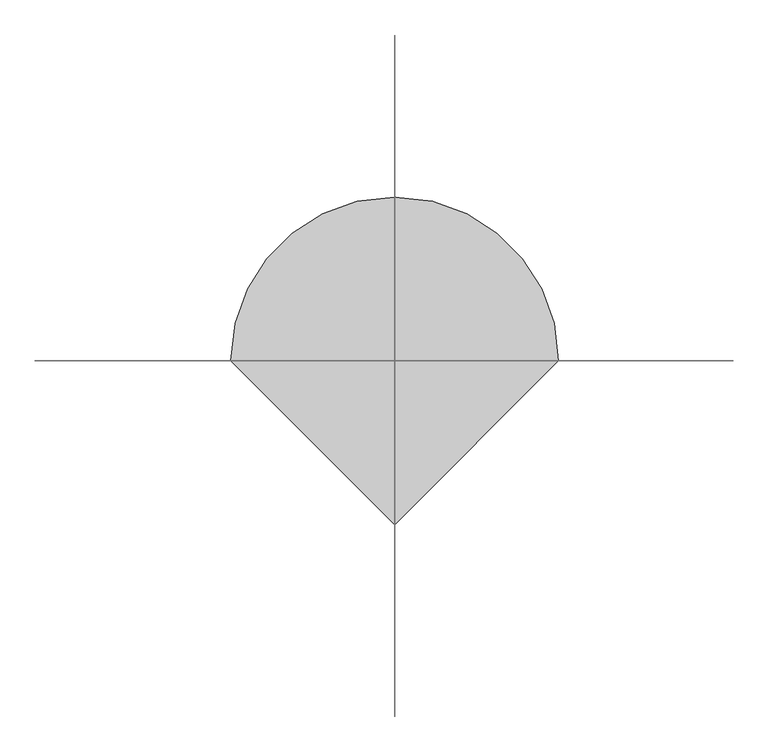
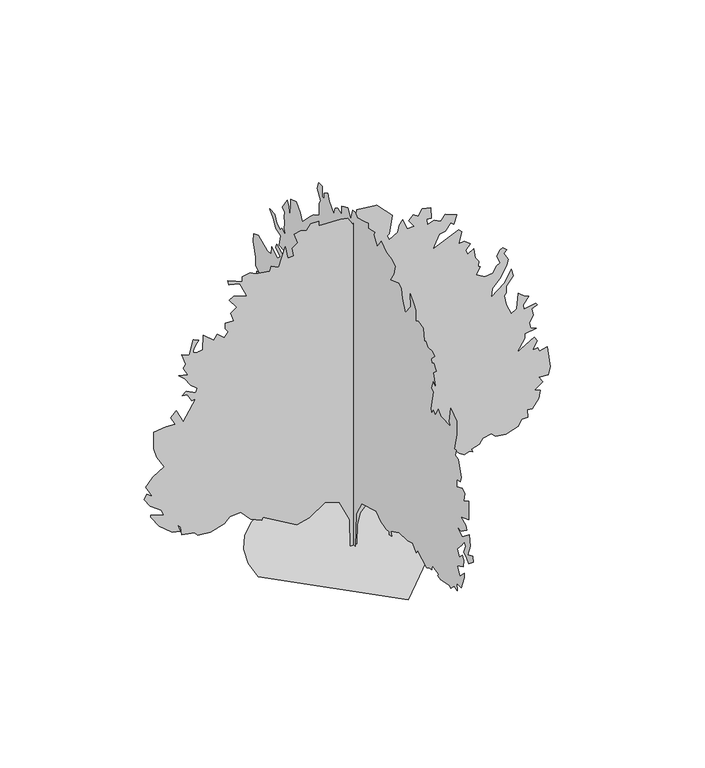
"""IFC4 building model written with IfcOpenShell, lengths in millimetres: proxy geometry, daphne 26070 : daphne 26070."""

import ifcopenshell
import ifcopenshell.guid

model = None  # the IFC model being written
_history = None  # IfcOwnerHistory: only IFC2X3 demands one
_inside = {}  # id of a spatial element -> (the spatial element, [elements in it])
_under = {}  # id of a project, library or spatial element -> (it, [spatial elements below it])
_declared = {}  # id of a project -> (the project, [libraries it declares])
_typed = {}  # id of a type object -> (the type object, [elements of that type])
_made_of = {}  # id of a material, layer set ... -> (it, [elements and type objects made of it])


def new_model(schema):
    """Start an empty IFC model of exactly this schema.

    Asked for "IFC4X3", IfcOpenShell would pick the latest addendum, in which some entities
    have other attributes; the version numbers below select the first issue.
    IFC2X3 requires an IfcOwnerHistory on every rooted entity: one is made here for all.
    """
    global model, _history
    if schema == "IFC4X3":
        model = ifcopenshell.file(schema_version=(4, 3, 0, 0))
    else:
        model = ifcopenshell.file(schema=schema)
    _inside.clear()
    _under.clear()
    _declared.clear()
    _typed.clear()
    _made_of.clear()
    _history = None
    if model.schema == "IFC2X3":
        org = make("IfcOrganization", Name="unknown")
        user = make(
            "IfcPersonAndOrganization",
            ThePerson=make("IfcPerson", FamilyName="unknown"),
            TheOrganization=org,
        )
        app = make(
            "IfcApplication",
            ApplicationDeveloper=org,
            Version="unknown",
            ApplicationFullName="unknown",
            ApplicationIdentifier="unknown",
        )
        _history = make(
            "IfcOwnerHistory",
            OwningUser=user,
            OwningApplication=app,
            ChangeAction="ADDED",
            CreationDate=0,
        )
    return model


def make(cls, **values):
    """One entity of the class cls with the attributes given. An attribute that is None is left unset."""
    return model.create_entity(
        cls, **{name: value for name, value in values.items() if value is not None}
    )


def rooted(cls, **values):
    """An entity with a GlobalId (a new one), such as an element, a storey or a relation."""
    return make(cls, GlobalId=ifcopenshell.guid.new(), OwnerHistory=_history, **values)


def si_unit(unit_type, name, prefix=None):
    """IfcSIUnit, for example si_unit("LENGTHUNIT", "METRE", prefix="MILLI")."""
    return make("IfcSIUnit", UnitType=unit_type, Prefix=prefix, Name=name)


def assignment(units):
    """IfcUnitAssignment: the units of a project."""
    return None if units is None else make("IfcUnitAssignment", Units=units)


def point(xyz):
    """IfcCartesianPoint."""
    return None if xyz is None else make("IfcCartesianPoint", Coordinates=xyz)


def direction(xyz):
    """IfcDirection."""
    return None if xyz is None else make("IfcDirection", DirectionRatios=xyz)


def frame(location, z_axis=None, x_axis=None):
    """IfcAxis2Placement3D, a coordinate frame: its origin and axes. An axis left out is left unset."""
    return make(
        "IfcAxis2Placement3D",
        Location=point(location),
        Axis=direction(z_axis),
        RefDirection=direction(x_axis),
    )


def origin():
    """The frame at (0, 0, 0) with its axes left unset."""
    return frame((0.0, 0.0, 0.0))


def place(relative_to, where):
    """IfcLocalPlacement: puts the frame where relative to a parent placement (None: the world)."""
    return make(
        "IfcLocalPlacement", PlacementRelTo=relative_to, RelativePlacement=where
    )


def context(
    kind, dimensions, precision=None, world=None, true_north=None, identifier=None
):
    """IfcGeometricRepresentationContext, for example the 3D "Model" context."""
    return make(
        "IfcGeometricRepresentationContext",
        ContextIdentifier=identifier,
        ContextType=kind,
        CoordinateSpaceDimension=dimensions,
        Precision=precision,
        WorldCoordinateSystem=world,
        TrueNorth=true_north,
    )


def project(units=None, contexts=None):
    """IfcProject with its units and contexts."""
    return rooted(
        "IfcProject",
        Name="project",
        RepresentationContexts=contexts,
        UnitsInContext=assignment(units),
    )


def spatial(cls, under=None, at=None, **own):
    """A site, building, storey or space (cls), placed at a placement, below another one or the project."""
    s = rooted(cls, ObjectPlacement=at, **own)
    if under is not None:
        _under.setdefault(under.id(), (under, []))[1].append(s)
    return s


def point_list(points):
    """IfcCartesianPointList2D or 3D."""
    cls = (
        "IfcCartesianPointList2D" if len(points[0]) == 2 else "IfcCartesianPointList3D"
    )
    return make(cls, CoordList=points)


def triangles(points, corners, closed=None, point_numbers=None):
    """IfcTriangulatedFaceSet: each triangle names its three corners, points numbered from 1."""
    return make(
        "IfcTriangulatedFaceSet",
        Coordinates=point_list(points),
        Closed=closed,
        CoordIndex=corners,
        PnIndex=point_numbers,
    )


def shape(context_of_items, identifier, shape_type, items):
    """IfcShapeRepresentation: the items that make up one representation, for example the "Body"."""
    return make(
        "IfcShapeRepresentation",
        ContextOfItems=context_of_items,
        RepresentationIdentifier=identifier,
        RepresentationType=shape_type,
        Items=items,
    )


def source(mapping_origin, context_of_items, identifier, shape_type, items):
    """IfcRepresentationMap: a shape defined once, which mapped items show again and again."""
    return make(
        "IfcRepresentationMap",
        MappingOrigin=mapping_origin,
        MappedRepresentation=shape(context_of_items, identifier, shape_type, items),
    )


def transform(
    local_origin,
    x_axis=None,
    y_axis=None,
    z_axis=None,
    scale=None,
    scale2=None,
    scale3=None,
    uniform=True,
):
    """IfcCartesianTransformationOperator3D, or its non-uniform kind. x_axis, y_axis, z_axis: its Axis1, 2, 3."""
    if uniform:
        return make(
            "IfcCartesianTransformationOperator3D",
            Axis1=direction(x_axis),
            Axis2=direction(y_axis),
            LocalOrigin=point(local_origin),
            Scale=scale,
            Axis3=direction(z_axis),
        )
    return make(
        "IfcCartesianTransformationOperator3DnonUniform",
        Axis1=direction(x_axis),
        Axis2=direction(y_axis),
        LocalOrigin=point(local_origin),
        Scale=scale,
        Axis3=direction(z_axis),
        Scale2=scale2,
        Scale3=scale3,
    )


def mapped(mapping_source, mapping_target):
    """IfcMappedItem: shows the shape of a source again, moved by a transform."""
    return make(
        "IfcMappedItem", MappingSource=mapping_source, MappingTarget=mapping_target
    )


def made_of(thing, what):
    """Note that an element or type object is made of a material, layer set ...; save() writes the relation."""
    if what is not None:
        _made_of.setdefault(what.id(), (what, []))[1].append(thing)
    return thing


def element(
    cls,
    number,
    at=None,
    inside=None,
    cuts=None,
    type_object=None,
    material=None,
    context=None,
    identifier="Body",
    shape_type=None,
    held_by="IfcProductDefinitionShape",
    body=None,
    shapes=None,
    **own,
):
    """One element of the class cls, such as IfcWall. Its Tag is "e" and its number.

    at: its placement. inside: the storey or other place that contains it. cuts: it is an
    opening in that element (IfcRelVoidsElement). A single representation is given by context,
    identifier, shape_type and body (its items); several are given by shapes. held_by: the class
    of the entity that holds the representations. save() writes the other relations.
    """
    e = rooted(cls, Tag="e%d" % number, ObjectPlacement=at, **own)
    if body is not None:
        shapes = [shape(context, identifier, shape_type, body)]
    if shapes is not None:
        e.Representation = make(held_by, Representations=shapes)
    if inside is not None:
        _inside.setdefault(inside.id(), (inside, []))[1].append(e)
    if cuts is not None:
        rooted(
            "IfcRelVoidsElement", RelatingBuildingElement=cuts, RelatedOpeningElement=e
        )
    if type_object is not None:
        _typed.setdefault(type_object.id(), (type_object, []))[1].append(e)
    return made_of(e, material)


def aggregate(whole, parts):
    """IfcRelAggregates: a whole, such as a stair, and the parts it consists of."""
    return rooted("IfcRelAggregates", RelatingObject=whole, RelatedObjects=parts)


def save(model, path):
    """Write the relations noted so far, then the file.

    IfcRelAggregates (storeys below a building ...), IfcRelContainedInSpatialStructure (elements
    in a storey), IfcRelDefinesByType, IfcRelAssociatesMaterial and IfcRelDeclares: one each for
    every whole, place, type object, material and project.
    """
    for whole, parts in _under.values():
        aggregate(whole, parts)
    for where, things in _inside.values():
        rooted(
            "IfcRelContainedInSpatialStructure",
            RelatedElements=things,
            RelatingStructure=where,
        )
    for kind, things in _typed.values():
        rooted("IfcRelDefinesByType", RelatedObjects=things, RelatingType=kind)
    for what, things in _made_of.values():
        rooted("IfcRelAssociatesMaterial", RelatedObjects=things, RelatingMaterial=what)
    for by, libraries in _declared.values():
        rooted("IfcRelDeclares", RelatingContext=by, RelatedDefinitions=libraries)
    model.write(path)


def entourage_98a115af(model_context):
    return source(origin(), model_context, "Body", "Tessellation", [
        triangles([(-9.4573925, 3.9e-06, 72.2348623), (-36.4693492, 6.1e-06, 128.8771626), (-74.629579, 5.2e-06, 141.2324949), (-113.9485589, 1.8e-06, 114.0498972), (-145.9624841, -1e-07, 106.0463523), (-234.001251, -8e-07, 158.0691489), (-236.002001, -1.4e-06, 150.0658583), (-264.0154255, -1.9e-06, 162.0709213), (-290.0250479, -1.3e-06, 190.0833467), (-318.0387268, -2.7e-06, 188.0823242), (-332.0443036, -4.1e-06, 174.0762387), (-368.4272936, -6.4e-06, 163.6409018), (-400.0731817, -7.6e-06, 166.0726938), (-408.0767266, -7.3e-06, 176.0772612), (-442.0924192, -8.5e-06, 182.0797836), (-444.0939686, -7.2e-06, 204.089414), (-452.0975135, -7.1e-06, 212.0929589), (-446.0929381, -7.9e-06, 194.0851191), (-466.1030903, -8.6e-06, 198.0868916), (-500.1187829, -8.4e-06, 226.0990444), (-522.1279046, -7.4e-06, 258.1124609), (-522.1279046, -7.1e-06, 264.1170363), (-488.1121757, -6.3e-06, 252.1104472), (-494.1142076, -5.6e-06, 268.117537), (-522.9229142, -5.6e-06, 288.9353979), (-538.1349944, -4.9e-06, 312.1357804), (-532.1304191, -3.9e-06, 324.1423513), (-518.1248423, -3.9e-06, 314.1372934), (-534.1319321, -2.8e-06, 344.14996), (-516.6084741, -8e-07, 365.2878413), (-486.7989927, 1.6e-06, 383.4742676), (-506.1208148, 2.7e-06, 416.1818642), (-514.1243597, 3.9e-06, 442.1940482), (-514.1243597, 6.5e-06, 486.2122553), (-482.1101801, 8.1e-06, 490.2153176), (-458.099509, 9.1e-06, 488.2138046), (-470.1035728, 9.9e-06, 510.2229263), (-456.097996, 1.13e-05, 524.2284668), (-438.0893932, 1e-05, 488.2138046), (-406.0752136, 1.45e-05, 540.2355566), (-416.0802715, 1.39e-05, 538.236587), (-428.0868788, 1.46e-05, 558.2441957), (-440.0909062, 1.42e-05, 560.2457088), (-430.0883918, 1.51e-05, 568.2492537), (-406.0752136, 1.54e-05, 556.2426827), (-401.4955876, 1.62e-05, 567.0275259), (-418.0817845, 1.63e-05, 580.2533175), (-434.0888743, 1.7e-05, 604.2639522), (-450.0959641, 1.72e-05, 618.2720724), (-426.0853294, 1.79e-05, 612.2674971), (-438.0893932, 1.87e-05, 634.2791622), (-432.0873613, 1.94e-05, 642.2826708), (-442.0924192, 2.07e-05, 672.2953737), (-422.0823034, 2.11e-05, 664.2917925), (-412.0797526, 2.38e-05, 702.308004), (-398.0716687, 2.41e-05, 696.3059721), (-400.6802304, 2.38e-05, 693.2783226), (-403.212634, 2.35e-05, 690.2023476), (-405.5926123, 2.32e-05, 687.0248526), (-407.7439708, 2.29e-05, 683.6948959), (-409.5930948, 2.26e-05, 680.1642975), (-411.0637536, 2.23e-05, 676.3821882), (-412.0797526, 2.21e-05, 672.2953737), (-411.9857903, 2.19e-05, 668.7317104), (-410.3525688, 2.18e-05, 666.420369), (-407.434106, 2.18e-05, 665.1452288), (-403.4920137, 2.2e-05, 664.7033226), (-398.7777666, 2.22e-05, 664.8861603), (-393.5530128, 2.25e-05, 665.485615), (-388.0691179, 2.28e-05, 666.2907984), (-386.0676049, 2.52e-05, 706.3085592), (-360.0554572, 2.49e-05, 682.2978882), (-350.0529064, 2.62e-05, 696.3059721), (-332.0443036, 2.6e-05, 680.2988823), (-322.0392457, 2.72e-05, 692.3029461), (-330.0427906, 2.76e-05, 704.3095533), (-330.0427906, 2.84e-05, 718.3150938), (-308.0336689, 2.94e-05, 718.3150938), (-316.0372138, 3.03e-05, 740.3242155), (-301.0029389, 3.16e-05, 751.5637184), (-320.0377327, 3.24e-05, 778.340427), (-308.0336689, 3.33e-05, 784.3424589), (-274.0179581, 3.42e-05, 774.3399445), (-292.0265791, 3.57e-05, 812.356156), (-320.9191106, 3.49e-05, 820.7254852), (-324.0407587, 3.54e-05, 832.3637283), (-304.0306247, 3.58e-05, 824.3602198), (-286.0245472, 3.62e-05, 816.3566385), (-286.0245472, 3.7e-05, 830.3647951), (-265.0619096, 3.8e-05, 832.6329706), (-252.0090908, 3.82e-05, 826.3616964), (-215.9931387, 3.95e-05, 820.3596645), (-211.9913662, 4.03e-05, 832.3637283), (-191.9827583, 4.06e-05, 822.3612139), (-175.9756504, 4.43e-05, 872.3814892), (-168.7203883, 4.27e-05, 839.3385933), (-153.9660381, 4.34e-05, 840.3673096), (-157.9678106, 4.45e-05, 862.3789747), (-143.9617251, 4.57e-05, 872.3814892), (-151.9650156, 4.69e-05, 898.3936369), (-135.9581802, 4.78e-05, 902.3941195), (-119.9513447, 4.83e-05, 898.3936369), (-109.9467864, 4.96e-05, 912.3991774), (-89.9381694, 5.05e-05, 912.3991774), (-89.9381694, 4.97e-05, 900.3951862), (-32.626833, 5.21e-05, 897.7739073), (-14.3439498, 5.26e-05, 893.5625364), (-1.8993678, 5.19e-05, 872.3814892), (6.1041838, 5.31e-05, 886.3895731), (8.105045, 5.45e-05, 908.3986948), (59.627565, 5.65e-05, 903.8140182), (99.4230465, 5.58e-05, 862.5999641), (92.1418776, 5.26e-05, 814.3577053), (86.1393461, 5.21e-05, 810.3546066), (92.1418776, 5.16e-05, 798.3505428), (114.1514989, 5.33e-05, 810.3546066), (118.1578496, 5.45e-05, 827.9416145), (126.1568253, 5.56e-05, 840.3673096), (138.1621427, 5.45e-05, 812.356156), (155.7905089, 5.52e-05, 811.8684677), (142.1639151, 5.58e-05, 832.3637283), (154.1689872, 5.71e-05, 844.3703356), (166.1743046, 5.71e-05, 836.3667543), (176.1785995, 5.85e-05, 852.3739168), (198.1884842, 5.92e-05, 848.3708181), (200.188998, 5.75e-05, 818.3581879), (188.1839168, 5.71e-05, 820.3596645), (190.1846849, 5.63e-05, 804.3525747), (208.1927972, 5.74e-05, 810.3546066), (224.199887, 5.76e-05, 802.3510981), (236.20495, 5.9e-05, 816.3566385), (265.7807247, 5.96e-05, 805.7293076), (258.2140718, 5.79e-05, 782.343453), (250.2110355, 5.79e-05, 788.3454849), (236.20495, 5.62e-05, 770.3369184), (220.1978602, 5.54e-05, 768.3379126), (204.1910248, 5.26e-05, 732.3207069), (270.2206608, 5.73e-05, 762.3333372), (278.2242057, 5.71e-05, 754.3298286), (270.2206608, 5.5e-05, 724.3171257), (284.2262195, 5.57e-05, 726.318675), (300.2333274, 5.57e-05, 714.3120678), (288.2267384, 5.43e-05, 700.3065273), (294.2312955, 5.39e-05, 688.3024635), (309.737998, 5.51e-05, 697.179756), (312.8444218, 5.37e-05, 671.3504459), (322.242431, 5.33e-05, 658.2872171), (320.240918, 5.25e-05, 646.283226), (326.2454933, 5.25e-05, 642.2801273), (316.2403991, 5.1e-05, 624.2741043), (337.7847236, 5.12e-05, 610.9797123), (358.2596729, 5.23e-05, 614.2690464), (368.2621874, 5.37e-05, 630.2761362), (378.0386619, 5.44e-05, 634.7135107), (368.2621874, 5.52e-05, 656.2882839), (376.2657323, 5.64e-05, 670.2938244), (384.2692772, 5.7e-05, 674.2943069), (394.2743714, 5.68e-05, 664.2917925), (386.2708265, 5.61e-05, 658.2872171), (398.1707179, 5.54e-05, 637.1290609), (394.2743714, 5.43e-05, 622.272555), (376.2657323, 5.17e-05, 592.2598884), (356.2581599, 4.97e-05, 572.2497725), (354.2566106, 4.83e-05, 550.2406508), (388.2723395, 5.13e-05, 576.2527986), (406.2783989, 5.4e-05, 608.2669782), (410.2814612, 5.3e-05, 588.2568624), (392.2728221, 5.09e-05, 566.2477407), (392.2728221, 4.98e-05, 548.2391015), (388.2723395, 4.93e-05, 542.2371059), (392.2728221, 4.79e-05, 516.2249219), (406.2783989, 4.67e-05, 486.2122553), (419.6692966, 4.79e-05, 495.1530613), (424.2870017, 5.05e-05, 536.235074), (440.2941278, 5.04e-05, 522.2294972), (450.2991858, 5.06e-05, 518.2264712), (437.047996, 4.89e-05, 500.1924339), (438.2925785, 4.83e-05, 488.2138046), (468.3077886, 4.99e-05, 494.2158002), (472.3083075, 4.97e-05, 488.2138046), (458.3027307, 4.88e-05, 482.2117727), (462.5902596, 4.78e-05, 462.3895815), (452.3006988, 4.64e-05, 446.1945308), (456.3012177, 4.56e-05, 430.187441), (470.3067581, 4.58e-05, 424.1854091), (440.2941278, 4.43e-05, 420.1849265), (440.2941278, 4.36e-05, 408.1783193), (420.2865191, 4.08e-05, 376.1641397), (464.3047626, 4.43e-05, 402.1762874), (472.3083075, 4.39e-05, 390.1697165), (460.3017002, 4.21e-05, 368.1605947), (474.3098205, 4.28e-05, 370.1621078), (478.3103394, 4.24e-05, 360.1570498), (498.3204552, 4.35e-05, 364.1600759), (506.3240001, 4.05e-05, 308.1352615), (500.3194247, 3.9e-05, 288.1251276), (476.3113335, 3.81e-05, 290.1266587), (486.3138843, 3.76e-05, 274.1195508), (464.3047626, 3.57e-05, 258.1124609), (480.3118524, 3.6e-05, 252.1104472), (476.3113335, 3.47e-05, 232.1015668), (460.3017002, 3.26e-05, 210.0919546), (446.2961234, 3.22e-05, 212.0929589), (448.2976727, 3.09e-05, 190.0833467), (432.2905829, 3.02e-05, 190.0833467), (424.2870017, 2.89e-05, 174.0762387), (391.7419679, 2.69e-05, 164.3614974), (366.2632178, 2.6e-05, 168.0737163), (354.2566106, 2.61e-05, 178.0780111), (332.2474889, 2.49e-05, 174.0762387), (323.8020015, 2.37e-05, 160.8723026), (302.2348404, 2.24e-05, 154.0673764), (306.2353412, 2.21e-05, 146.0640859), (298.2317963, 2.2e-05, 150.0658583), (284.2262195, 2.11e-05, 146.0640859), (272.2196304, 2.11e-05, 154.0673764), (260.2155848, 2.14e-05, 168.0737163), (240.2064682, 2.03e-05, 164.0719438), (236.8051496, 1.96e-05, 155.3752181), (196.1874799, 1.67e-05, 136.0595276), (196.1874799, 1.6e-05, 124.0544646), (162.1725321, 1.36e-05, 110.0481247), (162.1725321, 1.4e-05, 116.0509106), (138.1618883, 1.27e-05, 112.0491381), (106.7192036, 1.23e-05, 127.7984221), (83.214788, 1.13e-05, 128.4156446), (38.7434109, 8e-06, 104.983363), (17.3291135, 5.6e-06, 81.0641653), (9.1189377, 3.5e-06, 51.8726831), (8.1050195, 4e-07, 0.0), (-7.9020227, -3e-07, 7e-07), (-244.9072532, 0.0, 4.54e-05), (-238.4327937, 56.1165193, 4.18e-05), (-219.9933851, 107.6506239, 3.79e-05), (-191.0655541, 153.1257915, 3.39e-05), (-153.1257915, 191.0655541, 3e-05), (-107.6506239, 219.9933851, 2.63e-05), (-56.1165193, 238.4327937, 2.29e-05), (1.14e-05, 244.9072532, 2.01e-05), (56.1165193, 238.4327937, 1.8e-05), (107.6506239, 219.9933851, 5.12e-05), (153.1257915, 191.0655541, 5.1e-05), (191.0655541, 153.1257915, 5.16e-05), (219.9933851, 107.6506239, 1.87e-05), (238.4327937, 56.1165193, 2.09e-05), (244.9072532, -2.14e-05, 2.4e-05), (-3.16e-05, -244.9072532, 4.93e-05), (-1e-06, 8.7682648, 19.1210077), (-2.7e-06, 9.3654196, 78.8180451), (-6.1e-06, 33.2534526, 124.0544646), (-5.1e-06, 45.2590243, 110.0481247), (-5.2e-06, 55.2633328, 118.0516787), (-5.8e-06, 63.2666234, 112.0491381), (-6.9e-06, 91.2787853, 114.0498972), (-9e-06, 105.285116, 130.0569961), (-9.8e-06, 121.2919515, 126.0552236), (-9.6e-06, 133.2972779, 144.0630725), (-1.09e-05, 133.2972779, 162.0709213), (-1.16e-05, 181.318293, 146.0640859), (-1.37e-05, 187.3210879, 152.0666174), (-1.51e-05, 221.3357813, 154.0676308), (-1.31e-05, 215.3334951, 146.0640859), (-1.58e-05, 241.3446436, 158.0694032), (-1.53e-05, 243.3454117, 172.0754887), (-1.59e-05, 257.3504617, 172.0754887), (-1.75e-05, 259.3519928, 188.0825785), (-1.71e-05, 267.3555377, 204.089414), (-1.9e-05, 271.3585819, 214.0939814), (-1.92e-05, 297.3682044, 236.1036118), (-2.09e-05, 291.3661725, 240.1051299), (-2.09e-05, 315.3768253, 264.1170363), (-2.19e-05, 325.3818832, 250.1096791), (-2.19e-05, 331.3839151, 256.1134914), (-2.32e-05, 351.394031, 248.1086748), (-2.37e-05, 357.3960629, 242.1061342), (-2.46e-05, 381.4066976, 244.1069023), (-2.44e-05, 385.4072165, 254.1119602), (-2.53e-05, 409.4178512, 258.1124609), (-2.69e-05, 411.4193642, 272.1180377), (-2.71e-05, 423.423428, 278.1225949), (-2.96e-05, 455.4376076, 302.1332478), (-2.88e-05, 443.4335438, 310.1367745), (-3.05e-05, 469.4457278, 346.151473), (-3.18e-05, 465.4426655, 360.1570498), (-3.14e-05, 449.4355757, 354.1550179), (-3.05e-05, 445.4350931, 370.1621078), (-3.1e-05, 459.4406336, 374.1651701), (-3.29e-05, 474.5104623, 393.7968206), (-3.38e-05, 487.4517872, 434.1905033), (-3.29e-05, 443.4335438, 460.202651), (-3.07e-05, 433.4284859, 404.1778367), (-3e-05, 421.4244221, 408.1783193), (-3.36e-05, 431.6073034, 483.065209), (-3.29e-05, 419.4229091, 486.2122553), (-3.32e-05, 435.4299989, 496.2173495), (-3.43e-05, 435.4299989, 518.2264712), (-3.54e-05, 447.4340627, 554.2436769), (-3.64e-05, 443.4335438, 578.2543116), (-3.73e-05, 423.423428, 586.2578565), (-3.43e-05, 384.7290238, 566.6439737), (-3.35e-05, 367.3985773, 568.2492537), (-3.46e-05, 365.3996078, 590.2583754), (-3.2e-05, 339.38746, 574.2512856), (-3.09e-05, 325.3818832, 586.2578565), (-3.33e-05, 345.3894919, 600.2634333), (-3.26e-05, 341.388973, 610.2684912), (-3.2e-05, 313.375276, 596.2604073), (-3.12e-05, 309.3747934, 612.2674971), (-3.2e-05, 331.3839151, 614.2690464), (-3.26e-05, 324.6503509, 643.5704556), (-3.53e-05, 345.3894919, 652.2852579), (-3.49e-05, 357.3960629, 672.2953737), (-3.71e-05, 373.4031527, 688.3024635), (-3.62e-05, 351.394031, 686.3009142), (-3.44e-05, 341.388973, 668.2923477), (-3.42e-05, 327.3833962, 658.2897606), (-3.34e-05, 319.3798513, 668.2923477), (-3.31e-05, 301.3712485, 658.2897606), (-3.49e-05, 309.3747934, 674.2943069), (-3.4e-05, 305.3717311, 690.3013968), (-3.56e-05, 309.3747934, 706.3085592), (-3.5e-05, 307.3732804, 718.3150938), (-3.51e-05, 317.3783383, 726.318675), (-3.49e-05, 295.3692166, 758.3328547), (-3.52e-05, 289.3646595, 744.3272415), (-3.4e-05, 281.3610964, 716.3136171), (-3.58e-05, 279.3621268, 770.3369184), (-3.44e-05, 255.3514921, 778.340427), (-3.23e-05, 237.3428711, 760.334404), (-3.28e-05, 229.3393262, 740.3242155), (-3.11e-05, 209.330464, 760.334404), (-3.16e-05, 191.322606, 778.340427), (-3.05e-05, 177.3165205, 790.3470343), (-3.1e-05, 153.3061402, 804.3525747), (-3.17e-05, 153.3061402, 836.3667543), (-3.08e-05, 145.3025953, 848.3708181), (-3.26e-05, 161.3094307, 872.3814892), (-3.37e-05, 155.087445, 890.4942644), (-3.3e-05, 138.6373771, 891.588965), (-3.2e-05, 138.6373771, 863.4050749), (-3.17e-05, 129.7796238, 863.4050749), (-3.12e-05, 131.2962645, 876.3845152), (-3.22e-05, 115.28942, 886.3895731), (-3.04e-05, 107.2858751, 870.3824833), (-2.83e-05, 87.2770128, 848.3708181), (-2.94e-05, 81.2744813, 866.3794573), (-2.85e-05, 69.2691594, 874.3829659), (-2.82e-05, 53.2620651, 866.3794573), (-2.94e-05, 53.2620651, 888.388579), (-2.86e-05, 42.0070608, 894.8096987), (-2.75e-05, 25.2500576, 902.3966629), (-2.59e-05, 13.2446369, 878.3860645), (-2.63e-05, 3.2402807, 908.3986948), (-2.57e-05, -8.7649884, 910.4002441), (-2.58e-05, -16.768535, 900.3951862), (-2.39e-05, -50.7832783, 910.4002441), (-2.52e-05, -64.7893547, 914.4007267), (-2.37e-05, -64.7893547, 900.3951862), (-2.2e-05, -94.8025255, 908.3986948), (-2.26e-05, -90.8010074, 898.3936369), (-2.09e-05, -104.8068295, 874.3829659), (-2.11e-05, -122.8149417, 900.3951862), (-1.88e-05, -144.7590329, 883.3085838), (-1.79e-05, -169.2642141, 879.2750364), (-1.76e-05, -184.8420423, 870.3824833), (-1.68e-05, -179.1326343, 845.1882362), (-1.65e-05, -162.8324119, 820.3596645), (-1.63e-05, -200.8491321, 834.3652777), (-1.4e-05, -212.8544495, 826.3616964), (-1.49e-05, -216.8562219, 802.3510981), (-1.34e-05, -230.8623074, 772.3383951), (-1.32e-05, -254.871416, 802.3510981), (-1.4e-05, -252.8719378, 836.3667543), (-1.19e-05, -270.8810493, 816.3566385), (-1.21e-05, -276.8830812, 806.3541241), (-1.12e-05, -276.8830812, 778.340427), (-1.04e-05, -288.8871268, 784.3450024), (-9.7e-06, -310.8962485, 778.340427), (-8.7e-06, -314.8992745, 746.3262474), (-8.4e-06, -320.9013064, 748.3277967), (-6.3e-06, -330.9064007, 738.3227388), (-5.3e-06, -350.913973, 740.3242155), (-5.2e-06, -360.919031, 732.3207069), (-6.5e-06, -346.9134905, 716.3136171), (-4.7e-06, -348.9150035, 706.3085592), (-4.2e-06, -356.9185484, 710.3115852), (-4.3e-06, -368.9226122, 696.3059721), (-5.4e-06, -354.9170354, 684.2994375), (-4.1e-06, -364.9220933, 654.2867346), (-4.2e-06, -354.9170354, 662.2903158), (-3.5e-06, -346.9134905, 638.2796448), (-3.4e-06, -354.9170354, 632.2776129), (-1.8e-06, -344.9119411, 580.2533175), (-2.2e-06, -348.9150035, 568.2492537), (-1.3e-06, -354.9170354, 582.2548305), (-1.2e-06, -365.0364032, 574.0988966), (-1.8e-06, -376.9261571, 598.2619203), (4e-07, -388.932728, 586.2578565), (2.2e-06, -432.9509714, 584.2563435), (2.4e-06, -426.9489395, 594.2614014), (1e-07, -432.9509714, 634.2791622), (2.7e-06, -460.962125, 616.2705231), (3.1e-06, -458.9631191, 578.2543116), (5e-06, -448.9580612, 534.233561), (5.4e-06, -456.9616061, 534.233561), (4.5e-06, -453.2786187, 518.6607834), (5e-06, -466.966664, 516.2274653), (8e-06, -478.9707278, 474.2082278), (7.2e-06, -474.9702089, 460.202651), (6.5e-06, -460.962125, 458.201138), (7.6e-06, -458.9631191, 436.1920163), (9.3e-06, -484.9727597, 448.1960438), (9.4e-06, -495.8998544, 440.6471586), (1.04e-05, -490.9772987, 418.1833772), (9.7e-06, -512.9864204, 430.187441), (1.18e-05, -512.9864204, 380.167202), (9.6e-06, -476.9692148, 366.1616252), (1.23e-05, -498.9808436, 356.156531), (1.21e-05, -504.9828755, 346.151473), (1.23e-05, -478.9707278, 328.1428702), (1.17e-05, -462.963638, 330.1443832), (1.21e-05, -484.9727597, 316.1388064), (1.23e-05, -514.7745744, 340.233266), (1.35e-05, -520.9899653, 312.1357804), (1.38e-05, -508.9833944, 282.1231138), (1.52e-05, -530.9950596, 292.1281717), (1.67e-05, -532.7171565, 276.4538196), (1.52e-05, -513.8677983, 260.1292346), (1.52e-05, -504.9828755, 270.11905), (1.29e-05, -491.4116472, 278.5442443), (1.42e-05, -500.9798495, 300.1317166), (1.21e-05, -492.9763046, 308.1352615), (1.3e-05, -481.8053658, 291.1223283), (1.34e-05, -462.963638, 270.11905), (1.3e-05, -470.9671829, 252.1104472), (1.42e-05, -484.9727597, 266.1160058), (1.4e-05, -490.9772987, 256.1134914), (1.53e-05, -488.9757857, 238.1043617), (1.35e-05, -462.963638, 224.0982762), (1.52e-05, -472.9686959, 202.088664), (1.48e-05, -492.9763046, 222.0972719), (1.65e-05, -493.9364204, 210.9735868), (1.65e-05, -480.9722408, 176.0772612), (1.56e-05, -460.962125, 176.0772612), (1.7e-05, -462.963638, 156.0683989), (1.44e-05, -448.9580612, 160.0701714), (1.53e-05, -434.1422141, 145.3175835), (1.52e-05, -426.9489395, 150.0658583), (1.32e-05, -388.932728, 142.0623134), (1.26e-05, -374.9246078, 144.0630725), (1.31e-05, -378.9276701, 150.0658583), (1.21e-05, -350.913973, 156.0683989), (1.15e-05, -348.9150035, 144.0630725), (1.1e-05, -338.9099456, 142.0623134), (1.02e-05, -326.9033383, 136.0595276), (7.2e-06, -286.8856138, 158.0691489), (8.6e-06, -278.8845942, 148.0648449), (6.5e-06, -264.0916381, 164.6055958), (5.2e-06, -240.8666204, 158.0691489), (3.7e-06, -204.8506502, 158.0694032), (3.3e-06, -166.8341844, 138.060541), (3e-06, -170.8359568, 128.056237), (4.5e-06, -158.8306395, 124.0544646), (2.7e-06, -158.8306395, 132.0580095), (2e-06, -144.8243087, 130.0569961), (1.3e-06, -120.8141827, 138.060541), (-1e-06, -101.9528885, 154.2177488), (-2.5e-06, -36.7154756, 135.157575), (-1.1e-06, -12.638517, 93.3765678), (1.1e-06, -8.7649628, 3.52e-05), (3e-07, 9.2429405, 3.42e-05)], [[49, 48, 50], [95, 94, 96], [185, 184, 186], [213, 212, 214], [166, 165, 167], [167, 165, 168], [43, 42, 44], [53, 52, 54], [71, 70, 72], [44, 42, 45], [86, 85, 87], [85, 84, 87], [87, 84, 88], [42, 41, 45], [41, 40, 45], [174, 173, 175], [118, 117, 119], [18, 17, 19], [117, 116, 119], [145, 144, 146], [222, 221, 223], [22, 21, 23], [21, 20, 23], [133, 132, 134], [132, 131, 134], [131, 130, 134], [38, 37, 39], [37, 36, 39], [56, 55, 57], [165, 164, 168], [168, 164, 169], [169, 164, 170], [176, 175, 177], [175, 173, 177], [126, 125, 127], [180, 179, 181], [179, 178, 181], [177, 173, 178], [134, 130, 135], [135, 130, 136], [125, 124, 127], [124, 123, 127], [7, 6, 8], [27, 26, 28], [26, 25, 28], [81, 80, 82], [82, 80, 83], [158, 157, 159], [157, 156, 159], [156, 155, 159], [155, 154, 159], [159, 154, 160], [160, 154, 161], [93, 92, 94], [73, 72, 74], [204, 203, 205], [142, 141, 143], [194, 193, 195], [100, 99, 101], [57, 55, 58], [104, 103, 105], [77, 76, 78], [76, 75, 78], [110, 109, 111], [141, 140, 143], [101, 99, 102], [230, 229, 231], [231, 229, 1], [229, 228, 1], [189, 188, 190], [190, 188, 191], [198, 197, 199], [103, 102, 105], [149, 148, 150], [19, 17, 20], [20, 17, 23], [89, 88, 90], [161, 154, 162], [154, 153, 162], [153, 152, 162], [162, 152, 163], [152, 151, 163], [34, 33, 35], [1, 228, 2], [228, 227, 2], [84, 83, 88], [200, 199, 201], [48, 47, 50], [122, 121, 123], [121, 120, 123], [123, 120, 127], [127, 120, 128], [196, 195, 197], [195, 193, 197], [221, 220, 223], [192, 191, 193], [15, 14, 16], [79, 78, 80], [58, 55, 59], [55, 54, 59], [59, 54, 60], [60, 54, 61], [61, 54, 62], [62, 54, 63], [63, 54, 64], [64, 54, 65], [184, 183, 186], [130, 129, 136], [129, 128, 136], [138, 137, 139], [139, 137, 140], [88, 83, 90], [90, 83, 91], [91, 83, 92], [170, 164, 171], [29, 28, 30], [193, 191, 197], [191, 188, 197], [51, 50, 52], [25, 24, 28], [98, 97, 99], [111, 109, 112], [112, 109, 113], [113, 109, 114], [109, 108, 114], [136, 128, 137], [128, 120, 137], [202, 201, 203], [201, 199, 203], [181, 178, 182], [182, 178, 183], [35, 33, 36], [33, 32, 36], [32, 31, 36], [36, 31, 39], [120, 119, 137], [30, 28, 31], [54, 52, 65], [65, 52, 66], [52, 50, 66], [66, 50, 67], [67, 50, 68], [68, 50, 69], [119, 116, 137], [116, 115, 137], [173, 172, 178], [178, 172, 183], [183, 172, 186], [197, 188, 199], [28, 24, 31], [69, 50, 70], [215, 214, 216], [214, 212, 216], [216, 212, 217], [50, 47, 70], [47, 46, 70], [70, 46, 72], [72, 46, 74], [13, 12, 14], [206, 205, 207], [107, 106, 108], [140, 137, 143], [227, 226, 2], [147, 146, 148], [5, 4, 6], [4, 3, 6], [102, 99, 105], [99, 97, 105], [105, 97, 106], [106, 97, 108], [108, 97, 114], [114, 97, 115], [219, 218, 220], [143, 137, 144], [199, 188, 203], [203, 188, 205], [205, 188, 207], [207, 188, 208], [208, 188, 209], [209, 188, 210], [211, 210, 212], [212, 210, 217], [210, 188, 217], [217, 188, 218], [8, 6, 9], [80, 78, 83], [224, 223, 225], [223, 220, 225], [92, 83, 94], [12, 11, 14], [11, 10, 14], [14, 10, 16], [16, 10, 17], [17, 10, 23], [23, 10, 24], [24, 10, 31], [31, 10, 39], [10, 9, 39], [39, 9, 40], [9, 6, 40], [6, 3, 40], [40, 3, 45], [45, 3, 46], [46, 3, 74], [74, 3, 75], [75, 3, 78], [78, 3, 83], [83, 3, 94], [94, 3, 96], [96, 3, 97], [97, 3, 115], [115, 3, 137], [3, 2, 137], [2, 226, 137], [137, 226, 144], [144, 226, 146], [146, 226, 148], [148, 226, 150], [226, 225, 150], [225, 220, 150], [220, 218, 150], [218, 188, 150], [151, 150, 163], [163, 150, 164], [150, 188, 164], [164, 188, 171], [171, 188, 172], [172, 188, 186], [188, 187, 186], [247, 246, 232], [246, 245, 232], [232, 245, 233], [245, 244, 233], [233, 244, 234], [234, 244, 235], [244, 243, 235], [243, 242, 235], [235, 242, 236], [236, 242, 237], [237, 242, 238], [238, 242, 239], [239, 242, 240], [240, 242, 241], [262, 261, 263], [389, 388, 390], [373, 372, 374], [313, 312, 314], [441, 440, 442], [442, 440, 443], [314, 312, 315], [312, 311, 315], [359, 358, 360], [324, 323, 325], [415, 414, 416], [423, 422, 424], [302, 301, 303], [450, 449, 451], [401, 400, 402], [402, 400, 403], [400, 399, 403], [445, 444, 446], [315, 311, 316], [311, 310, 316], [290, 289, 291], [289, 288, 291], [288, 287, 291], [287, 286, 291], [281, 280, 282], [397, 396, 398], [323, 322, 325], [325, 322, 326], [463, 462, 464], [462, 461, 464], [426, 425, 427], [427, 425, 428], [428, 425, 429], [443, 440, 444], [269, 268, 270], [357, 356, 358], [395, 394, 396], [436, 435, 437], [437, 435, 438], [438, 435, 439], [429, 425, 430], [430, 425, 431], [425, 424, 431], [405, 404, 406], [374, 372, 375], [375, 372, 376], [457, 456, 458], [272, 271, 273], [372, 371, 376], [416, 414, 417], [309, 308, 310], [343, 342, 344], [342, 341, 344], [306, 305, 307], [305, 304, 307], [284, 283, 285], [283, 282, 285], [339, 338, 340], [338, 337, 340], [337, 336, 340], [362, 361, 363], [383, 382, 384], [382, 381, 384], [471, 470, 248], [470, 469, 248], [248, 469, 249], [249, 469, 250], [469, 468, 250], [387, 386, 388], [386, 385, 388], [403, 399, 404], [251, 250, 252], [351, 350, 352], [419, 418, 420], [418, 417, 420], [420, 417, 421], [322, 321, 326], [321, 320, 326], [293, 292, 294], [265, 264, 266], [317, 316, 318], [316, 310, 318], [310, 308, 318], [447, 446, 448], [431, 424, 432], [424, 422, 432], [432, 422, 433], [365, 364, 366], [278, 277, 279], [263, 261, 264], [256, 255, 257], [399, 398, 404], [327, 326, 328], [328, 326, 329], [329, 326, 330], [453, 452, 454], [398, 396, 404], [413, 412, 414], [412, 411, 414], [414, 411, 417], [378, 377, 379], [377, 376, 379], [340, 336, 341], [409, 408, 410], [344, 341, 345], [422, 421, 433], [433, 421, 434], [364, 363, 366], [366, 363, 367], [363, 361, 367], [408, 407, 410], [407, 406, 410], [392, 391, 393], [341, 336, 345], [257, 255, 258], [259, 258, 260], [380, 379, 381], [276, 275, 277], [275, 274, 277], [353, 352, 354], [354, 352, 355], [349, 348, 350], [350, 348, 352], [347, 346, 348], [346, 345, 348], [298, 297, 299], [299, 297, 300], [297, 296, 300], [295, 294, 296], [296, 294, 300], [300, 294, 301], [336, 335, 345], [335, 334, 345], [455, 454, 456], [454, 452, 456], [360, 358, 361], [368, 367, 369], [369, 367, 370], [291, 286, 292], [356, 355, 358], [449, 448, 451], [440, 439, 444], [404, 396, 406], [396, 394, 406], [406, 394, 410], [410, 394, 411], [376, 371, 379], [370, 367, 371], [301, 294, 303], [254, 253, 255], [253, 252, 255], [294, 292, 303], [319, 318, 320], [320, 318, 326], [326, 318, 330], [435, 434, 439], [355, 352, 358], [358, 352, 361], [361, 352, 367], [261, 260, 264], [417, 411, 421], [411, 394, 421], [255, 252, 258], [252, 250, 258], [352, 348, 367], [348, 345, 367], [345, 334, 367], [367, 334, 371], [334, 333, 371], [333, 332, 371], [332, 331, 371], [331, 330, 371], [330, 318, 371], [318, 308, 371], [308, 307, 371], [371, 307, 379], [379, 307, 381], [381, 307, 384], [384, 307, 385], [385, 307, 388], [388, 307, 390], [390, 307, 391], [391, 307, 393], [393, 307, 394], [394, 307, 421], [421, 307, 434], [434, 307, 439], [439, 307, 444], [444, 307, 446], [446, 307, 448], [448, 307, 451], [451, 307, 452], [452, 307, 456], [456, 307, 458], [458, 307, 459], [459, 307, 460], [460, 307, 461], [461, 307, 464], [464, 307, 465], [465, 307, 466], [466, 307, 467], [467, 307, 468], [468, 307, 250], [250, 307, 258], [307, 304, 258], [304, 303, 258], [303, 292, 258], [258, 292, 260], [274, 273, 277], [277, 273, 279], [273, 271, 279], [280, 279, 282], [279, 271, 282], [282, 271, 285], [285, 271, 286], [286, 271, 292], [292, 271, 260], [271, 270, 260], [270, 268, 260], [260, 268, 264], [264, 268, 266], [266, 268, 267]], closed=False),
    ])


if __name__ == "__main__":
    model = new_model("IFC4")
    model_context = context("Model", 3, world=origin())
    ifc_project = project(units=[si_unit("LENGTHUNIT", "METRE", prefix="MILLI")], contexts=[model_context])
    site = spatial("IfcSite", under=ifc_project)
    building = spatial("IfcBuilding", under=site)
    placement = place(None, origin())
    entourage_shape = entourage_98a115af(model_context)
    element("IfcBuildingElementProxy", 1, Name="daphne 26070 : daphne 26070", ObjectType="daphne 26070 : daphne 26070", at=placement, inside=building, context=model_context, shape_type="MappedRepresentation", body=[
        mapped(entourage_shape, transform((0.0, 0.0, 0.0), x_axis=(1.0, 0.0, 0.0), y_axis=(0.0, 1.0, 0.0), z_axis=(0.0, 0.0, 1.0))),
    ])
    save(model, "model.ifc")

# Revit data of these elements
# Type "daphne 26070 : daphne 26070"
#   built-in parameter 1005195 = "RPC-16-FUMB-EMQ0-U9RG-4000-ST1L-LVER-AU"
#   Height = 0
